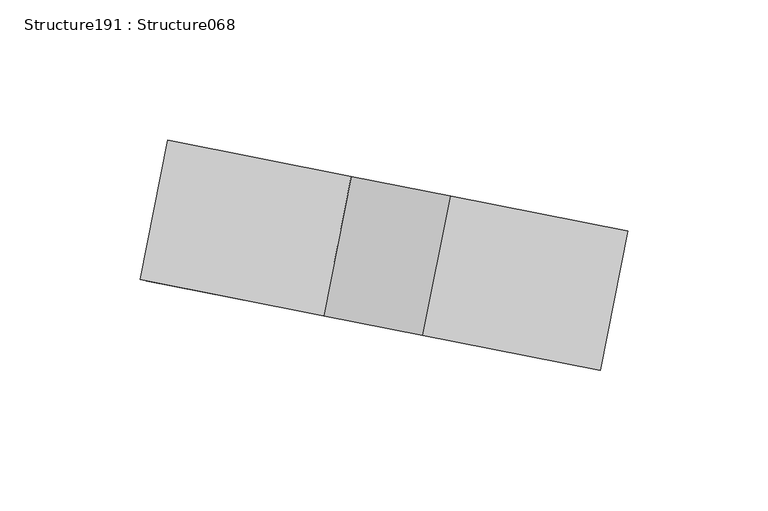
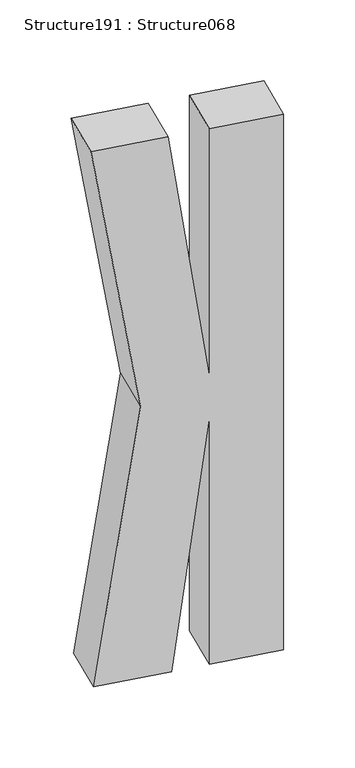
"""IFC4 building model written with IfcOpenShell, lengths in millimetres: proxy geometry, Structure191 : Structure068."""

import ifcopenshell
import ifcopenshell.guid

model = None  # the IFC model being written
_history = None  # IfcOwnerHistory: only IFC2X3 demands one
_inside = {}  # id of a spatial element -> (the spatial element, [elements in it])
_under = {}  # id of a project, library or spatial element -> (it, [spatial elements below it])
_declared = {}  # id of a project -> (the project, [libraries it declares])
_typed = {}  # id of a type object -> (the type object, [elements of that type])
_made_of = {}  # id of a material, layer set ... -> (it, [elements and type objects made of it])


def new_model(schema):
    """Start an empty IFC model of exactly this schema.

    Asked for "IFC4X3", IfcOpenShell would pick the latest addendum, in which some entities
    have other attributes; the version numbers below select the first issue.
    IFC2X3 requires an IfcOwnerHistory on every rooted entity: one is made here for all.
    """
    global model, _history
    if schema == "IFC4X3":
        model = ifcopenshell.file(schema_version=(4, 3, 0, 0))
    else:
        model = ifcopenshell.file(schema=schema)
    _inside.clear()
    _under.clear()
    _declared.clear()
    _typed.clear()
    _made_of.clear()
    _history = None
    if model.schema == "IFC2X3":
        org = make("IfcOrganization", Name="unknown")
        user = make(
            "IfcPersonAndOrganization",
            ThePerson=make("IfcPerson", FamilyName="unknown"),
            TheOrganization=org,
        )
        app = make(
            "IfcApplication",
            ApplicationDeveloper=org,
            Version="unknown",
            ApplicationFullName="unknown",
            ApplicationIdentifier="unknown",
        )
        _history = make(
            "IfcOwnerHistory",
            OwningUser=user,
            OwningApplication=app,
            ChangeAction="ADDED",
            CreationDate=0,
        )
    return model


def make(cls, **values):
    """One entity of the class cls with the attributes given. An attribute that is None is left unset."""
    return model.create_entity(
        cls, **{name: value for name, value in values.items() if value is not None}
    )


def rooted(cls, **values):
    """An entity with a GlobalId (a new one), such as an element, a storey or a relation."""
    return make(cls, GlobalId=ifcopenshell.guid.new(), OwnerHistory=_history, **values)


def si_unit(unit_type, name, prefix=None):
    """IfcSIUnit, for example si_unit("LENGTHUNIT", "METRE", prefix="MILLI")."""
    return make("IfcSIUnit", UnitType=unit_type, Prefix=prefix, Name=name)


def assignment(units):
    """IfcUnitAssignment: the units of a project."""
    return None if units is None else make("IfcUnitAssignment", Units=units)


def point(xyz):
    """IfcCartesianPoint."""
    return None if xyz is None else make("IfcCartesianPoint", Coordinates=xyz)


def direction(xyz):
    """IfcDirection."""
    return None if xyz is None else make("IfcDirection", DirectionRatios=xyz)


def frame(location, z_axis=None, x_axis=None):
    """IfcAxis2Placement3D, a coordinate frame: its origin and axes. An axis left out is left unset."""
    return make(
        "IfcAxis2Placement3D",
        Location=point(location),
        Axis=direction(z_axis),
        RefDirection=direction(x_axis),
    )


def origin():
    """The frame at (0, 0, 0) with its axes left unset."""
    return frame((0.0, 0.0, 0.0))


def place(relative_to, where):
    """IfcLocalPlacement: puts the frame where relative to a parent placement (None: the world)."""
    return make(
        "IfcLocalPlacement", PlacementRelTo=relative_to, RelativePlacement=where
    )


def context(
    kind, dimensions, precision=None, world=None, true_north=None, identifier=None
):
    """IfcGeometricRepresentationContext, for example the 3D "Model" context."""
    return make(
        "IfcGeometricRepresentationContext",
        ContextIdentifier=identifier,
        ContextType=kind,
        CoordinateSpaceDimension=dimensions,
        Precision=precision,
        WorldCoordinateSystem=world,
        TrueNorth=true_north,
    )


def project(units=None, contexts=None):
    """IfcProject with its units and contexts."""
    return rooted(
        "IfcProject",
        Name="project",
        RepresentationContexts=contexts,
        UnitsInContext=assignment(units),
    )


def spatial(cls, under=None, at=None, **own):
    """A site, building, storey or space (cls), placed at a placement, below another one or the project."""
    s = rooted(cls, ObjectPlacement=at, **own)
    if under is not None:
        _under.setdefault(under.id(), (under, []))[1].append(s)
    return s


def polyline(points):
    """IfcPolyline through the points."""
    return make("IfcPolyline", Points=[point(p) for p in points])


def outline(outer, holes=None, kind="AREA"):
    """IfcArbitraryClosedProfileDef: a profile drawn as a closed curve; with holes, ...WithVoids."""
    if holes is None:
        return make("IfcArbitraryClosedProfileDef", ProfileType=kind, OuterCurve=outer)
    return make(
        "IfcArbitraryProfileDefWithVoids",
        ProfileType=kind,
        OuterCurve=outer,
        InnerCurves=holes,
    )


def extrude(swept, where, along, depth):
    """IfcExtrudedAreaSolid: the profile swept, set in the frame where, extruded along a direction by depth."""
    return make(
        "IfcExtrudedAreaSolid",
        SweptArea=swept,
        Position=where,
        ExtrudedDirection=direction(along),
        Depth=depth,
    )


def shape(context_of_items, identifier, shape_type, items):
    """IfcShapeRepresentation: the items that make up one representation, for example the "Body"."""
    return make(
        "IfcShapeRepresentation",
        ContextOfItems=context_of_items,
        RepresentationIdentifier=identifier,
        RepresentationType=shape_type,
        Items=items,
    )


def source(mapping_origin, context_of_items, identifier, shape_type, items):
    """IfcRepresentationMap: a shape defined once, which mapped items show again and again."""
    return make(
        "IfcRepresentationMap",
        MappingOrigin=mapping_origin,
        MappedRepresentation=shape(context_of_items, identifier, shape_type, items),
    )


def transform(
    local_origin,
    x_axis=None,
    y_axis=None,
    z_axis=None,
    scale=None,
    scale2=None,
    scale3=None,
    uniform=True,
):
    """IfcCartesianTransformationOperator3D, or its non-uniform kind. x_axis, y_axis, z_axis: its Axis1, 2, 3."""
    if uniform:
        return make(
            "IfcCartesianTransformationOperator3D",
            Axis1=direction(x_axis),
            Axis2=direction(y_axis),
            LocalOrigin=point(local_origin),
            Scale=scale,
            Axis3=direction(z_axis),
        )
    return make(
        "IfcCartesianTransformationOperator3DnonUniform",
        Axis1=direction(x_axis),
        Axis2=direction(y_axis),
        LocalOrigin=point(local_origin),
        Scale=scale,
        Axis3=direction(z_axis),
        Scale2=scale2,
        Scale3=scale3,
    )


def mapped(mapping_source, mapping_target):
    """IfcMappedItem: shows the shape of a source again, moved by a transform."""
    return make(
        "IfcMappedItem", MappingSource=mapping_source, MappingTarget=mapping_target
    )


def made_of(thing, what):
    """Note that an element or type object is made of a material, layer set ...; save() writes the relation."""
    if what is not None:
        _made_of.setdefault(what.id(), (what, []))[1].append(thing)
    return thing


def element(
    cls,
    number,
    at=None,
    inside=None,
    cuts=None,
    type_object=None,
    material=None,
    context=None,
    identifier="Body",
    shape_type=None,
    held_by="IfcProductDefinitionShape",
    body=None,
    shapes=None,
    **own,
):
    """One element of the class cls, such as IfcWall. Its Tag is "e" and its number.

    at: its placement. inside: the storey or other place that contains it. cuts: it is an
    opening in that element (IfcRelVoidsElement). A single representation is given by context,
    identifier, shape_type and body (its items); several are given by shapes. held_by: the class
    of the entity that holds the representations. save() writes the other relations.
    """
    e = rooted(cls, Tag="e%d" % number, ObjectPlacement=at, **own)
    if body is not None:
        shapes = [shape(context, identifier, shape_type, body)]
    if shapes is not None:
        e.Representation = make(held_by, Representations=shapes)
    if inside is not None:
        _inside.setdefault(inside.id(), (inside, []))[1].append(e)
    if cuts is not None:
        rooted(
            "IfcRelVoidsElement", RelatingBuildingElement=cuts, RelatedOpeningElement=e
        )
    if type_object is not None:
        _typed.setdefault(type_object.id(), (type_object, []))[1].append(e)
    return made_of(e, material)


def aggregate(whole, parts):
    """IfcRelAggregates: a whole, such as a stair, and the parts it consists of."""
    return rooted("IfcRelAggregates", RelatingObject=whole, RelatedObjects=parts)


def save(model, path):
    """Write the relations noted so far, then the file.

    IfcRelAggregates (storeys below a building ...), IfcRelContainedInSpatialStructure (elements
    in a storey), IfcRelDefinesByType, IfcRelAssociatesMaterial and IfcRelDeclares: one each for
    every whole, place, type object, material and project.
    """
    for whole, parts in _under.values():
        aggregate(whole, parts)
    for where, things in _inside.values():
        rooted(
            "IfcRelContainedInSpatialStructure",
            RelatedElements=things,
            RelatingStructure=where,
        )
    for kind, things in _typed.values():
        rooted("IfcRelDefinesByType", RelatedObjects=things, RelatingType=kind)
    for what, things in _made_of.values():
        rooted("IfcRelAssociatesMaterial", RelatedObjects=things, RelatingMaterial=what)
    for by, libraries in _declared.values():
        rooted("IfcRelDeclares", RelatingContext=by, RelatedDefinitions=libraries)
    model.write(path)


def structure191_structure068_1e06ae66(model_context):
    return source(origin(), model_context, "Body", "SweptSolid", [
        extrude(outline(polyline([(274.9994632, -1e-07), (264.9886589, -66.8596997), (13.921021, -62.6677254), (260.0973798, -99.5273491), (250.5395907, -163.3614715), (-281.3127819, -83.7279989), (-271.7549927, -19.8938765), (-24.8238231, -56.8665169), (-266.4085382, 15.8137778), (-256.511172, 81.9158516), (0.0, 0.0), (274.9994632, -1e-07)])), frame((-2264.2411627, 234917.8361746, 867.171671), z_axis=(0.19466222296394126, 0.9808703374813295, 0.0), x_axis=(-0.14524519607623845, 0.02882516848825376, -0.988975703785689)), (0.0, 0.0, 1.0), 50.8),
    ])


if __name__ == "__main__":
    model = new_model("IFC4")
    model_context = context("Model", 3, world=origin())
    ifc_project = project(units=[si_unit("LENGTHUNIT", "METRE", prefix="MILLI")], contexts=[model_context])
    site = spatial("IfcSite", under=ifc_project)
    building = spatial("IfcBuilding", under=site)
    placement = place(None, origin())
    structure191_structure068_shape = structure191_structure068_1e06ae66(model_context)
    element("IfcBuildingElementProxy", 1, Name="Structure191 : Structure068", ObjectType="Structure191 : Structure068", at=placement, inside=building, context=model_context, shape_type="MappedRepresentation", body=[
        mapped(structure191_structure068_shape, transform((0.0, 0.0, 0.0), x_axis=(1.0, 0.0, 0.0), y_axis=(0.0, 1.0, 0.0), z_axis=(0.0, 0.0, 1.0))),
    ])
    save(model, "model.ifc")

# Revit data of these elements
# Type "Structure191 : Structure068"
#   NameOverride = "Structure068"
# Element 1 (IfcBuildingElementProxy, "Structure191 : Structure068")
#   Materials on its faces: "BRUSHED ALUMINUM LETTERING"
# Materials
#   "BRUSHED ALUMINUM LETTERING": class "Unassigned", colour RGB 169 181 186, transparency 0, Cost = 0
